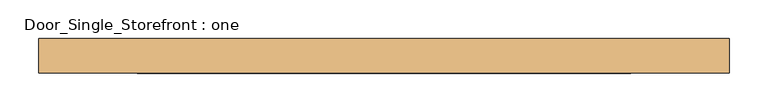
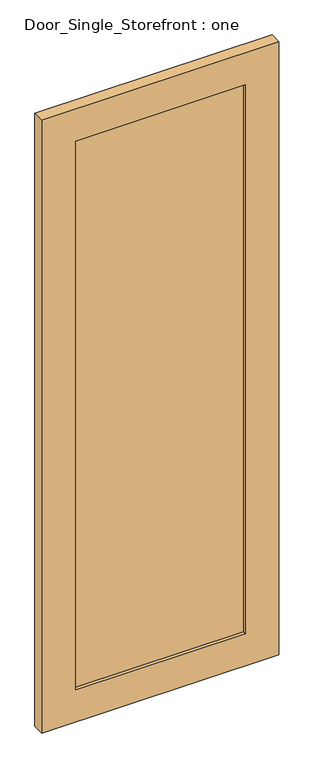
"""IFC4 building model written with IfcOpenShell, lengths in millimetres: door geometry, Door_Single_Storefront : one."""

from ifc_helpers import new_model, si_unit, frame, origin, place, context, project, spatial, polyline, outline, extrude, source, transform, mapped, element, save


def door_single_storefront_one_9b1c4f31(model_context):
    return source(origin(), model_context, "Body", "SweptSolid", [
        extrude(outline(polyline([(318.29375, 6.35), (318.29375, -12.7), (-318.29375, -12.7), (-318.29375, 6.35), (318.29375, 6.35)])), frame((0.0, 0.0, 127.0), z_axis=(0.0, 0.0, 1.0), x_axis=(1.0, 0.0, 0.0)), (0.0, 0.0, 1.0), 2178.05),
        extrude(outline(polyline([(2432.05, -445.29375), (0.0, -445.29375), (0.0, 445.29375), (2432.05, 445.29375), (2432.05, -445.29375)]), holes=[polyline([(127.0, 318.29375), (127.0, -318.29375), (2305.05, -318.29375), (2305.05, 318.29375), (127.0, 318.29375)])]), frame((0.0, -25.4, 0.0), z_axis=(0.0, 1.0, 0.0), x_axis=(0.0, 0.0, 1.0)), (0.0, 0.0, 1.0), 44.45),
    ])


if __name__ == "__main__":
    model = new_model("IFC4")
    model_context = context("Model", 3, world=origin())
    ifc_project = project(units=[si_unit("LENGTHUNIT", "METRE", prefix="MILLI")], contexts=[model_context])
    site = spatial("IfcSite", under=ifc_project)
    building = spatial("IfcBuilding", under=site)
    placement = place(None, origin())
    door_single_storefront_one_shape = door_single_storefront_one_9b1c4f31(model_context)
    element("IfcDoor", 1, ObjectType="Door_Single_Storefront : one", at=placement, inside=building, context=model_context, shape_type="MappedRepresentation", body=[
        mapped(door_single_storefront_one_shape, transform((0.0, 0.0, 0.0), x_axis=(1.0, 0.0, 0.0), y_axis=(0.0, 1.0, 0.0), z_axis=(0.0, 0.0, 1.0))),
    ])
    save(model, "model.ifc")

# Revit data of these elements
# Type "Door_Single_Storefront : one"
#   Type Mark = "27"
#   Analytic Construction = "<None>"
#   Stile_Width = 0' - 5"
#   Door_Thickness = 0' - 1 3/4"
#   Door_Offset = 0' - 1"
#   Glass_Material = SAFETY GLAZING
#   Frame_Material = INTERIOR GRADE ALUMINUM STOREFRONT W/ SAFETY GLAZING
#   Function = (empty or 0)
# Element 1 (IfcDoor, "Door_Single_Storefront : one")
#   Materials on its faces: "INTERIOR GRADE ALUMINUM STOREFRONT W/ SAFETY GLAZING", "SAFETY GLAZING"
# Materials
#   "SAFETY GLAZING": class "Glass", colour RGB 142 168 196, transparency 0.75, Description = "Soda Lime Glass", Cost = 0
#   "INTERIOR GRADE ALUMINUM STOREFRONT W/ SAFETY GLAZING": class "Metal", colour RGB 226 226 226, transparency 0, Description = "Aluminum 6061", Cost = 0
